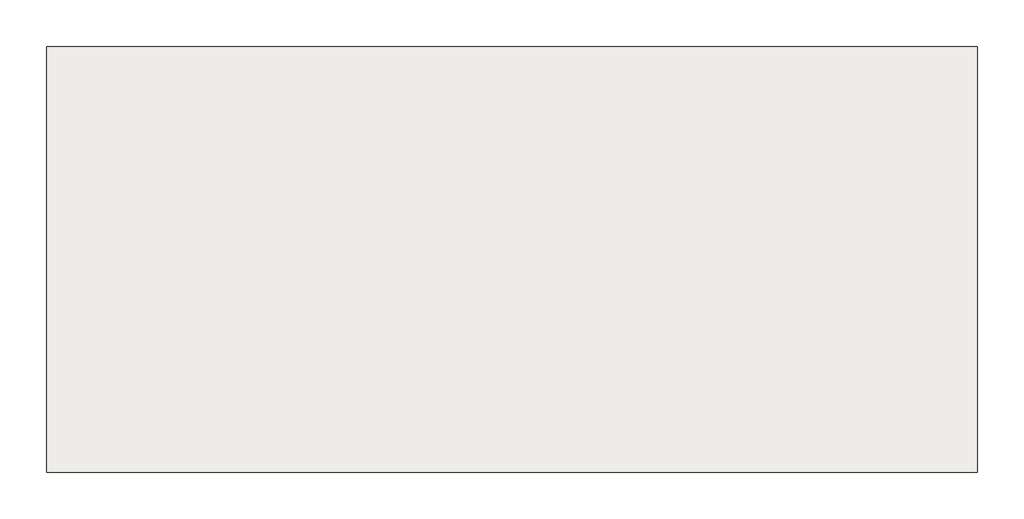
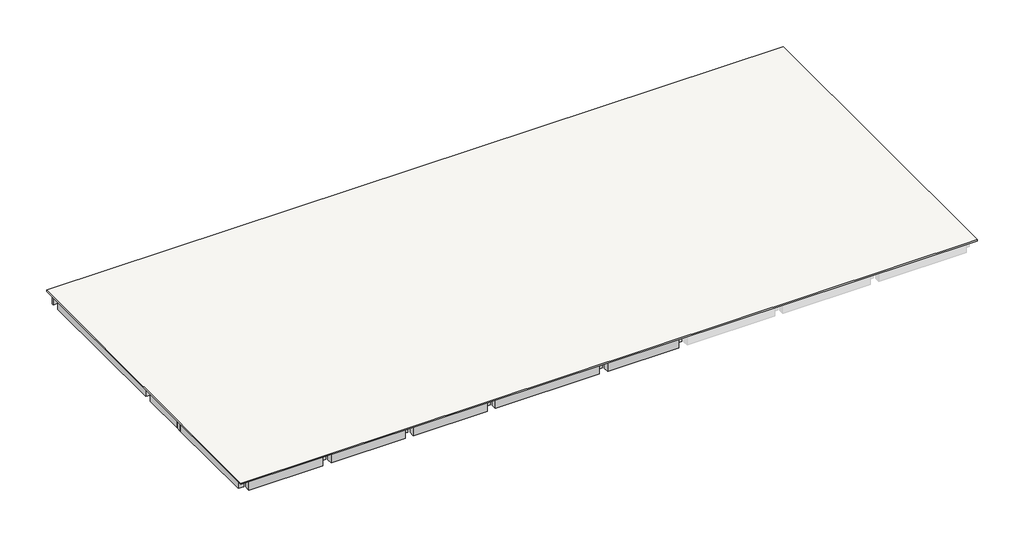
# One storey, part 1 of 2: 29 beams, 1 roof.
"""IFC4 building model written with IfcOpenShell, lengths in millimetres."""

from ifc_helpers import new_model, si_unit, frame, origin, place, context, project, spatial, polyline, outline, extrude, faceted_brep, element, save

model = new_model("IFC4")

# Units and contexts
model_context = context("Model", 3, world=origin())
ifc_project = project(units=[si_unit("LENGTHUNIT", "METRE", prefix="MILLI")], contexts=[model_context])

# Site, building, storey
site = spatial("IfcSite", under=ifc_project)
building = spatial("IfcBuilding", under=site)
storey = spatial("IfcBuildingStorey", under=building, Name="TOC", Elevation=7650.0)

# Beams
placement = place(None, origin())
element("IfcBeam", 1, ObjectType="RC Beam_Rectangular : H_SB_ACB_B400xH900", at=placement, inside=storey, context=model_context, shape_type="Brep", body=[
    faceted_brep([(224.7, 12116.5208589, 7500.0), (224.7, 12116.5208589, 6750.0), (5624.7, 12116.5208589, 6750.0), (5624.7, 12116.5208589, 7500.0), (5724.7, 12116.5208589, 7500.0), (6124.7, 12116.5208589, 7500.0), (6124.7, 12116.5208589, 7549.0), (5724.7, 12116.5208589, 7549.0), (124.7, 12116.5208589, 7549.0), (-275.3, 12116.5208589, 7549.0), (-275.3, 12116.5208589, 7500.0), (124.7, 12116.5208589, 7500.0), (224.7, 12516.5208589, 6750.0), (5624.7, 12516.5208589, 6750.0), (224.7, 12516.5208589, 7500.0), (124.7, 12516.5208589, 7500.0), (-275.3, 12516.5208589, 7500.0), (-275.3, 12516.5208589, 7549.0), (124.7, 12516.5208589, 7549.0), (5724.7, 12516.5208589, 7549.0), (6124.7, 12516.5208589, 7549.0), (6124.7, 12516.5208589, 7500.0), (5724.7, 12516.5208589, 7500.0), (5624.7, 12516.5208589, 7500.0)], [[[0, 1, 2, 3, 4, 5, 6, 7, 8, 9, 10, 11]], [[1, 12, 13, 2]], [[12, 14, 15, 16, 17, 18, 19, 20, 21, 22, 23, 13]], [[1, 0, 14, 12]], [[0, 11, 10, 16, 15, 14]], [[23, 3, 2, 13]], [[3, 23, 22, 21, 5, 4]], [[9, 8, 7, 6, 20, 19, 18, 17]], [[9, 17, 16, 10]], [[20, 6, 5, 21]]]),
])
element("IfcBeam", 2, ObjectType="RC Beam_Rectangular : H_SB_ACB_B400xH900", at=placement, inside=storey, context=model_context, shape_type="Brep", body=[
    faceted_brep([(6224.7, 12116.5208589, 7500.0), (6224.7, 12116.5208589, 6750.0), (11624.7, 12116.5208589, 6750.0), (11624.7, 12116.5208589, 7500.0), (11724.7, 12116.5208589, 7500.0), (12124.7, 12116.5208589, 7500.0), (12124.7, 12116.5208589, 7549.0), (11724.7, 12116.5208589, 7549.0), (6124.7, 12116.5208589, 7549.0), (6124.7, 12116.5208589, 7500.0), (6224.7, 12516.5208589, 6750.0), (11624.7, 12516.5208589, 6750.0), (6224.7, 12516.5208589, 7500.0), (6124.7, 12516.5208589, 7500.0), (6124.7, 12516.5208589, 7549.0), (11724.7, 12516.5208589, 7549.0), (12124.7, 12516.5208589, 7549.0), (12124.7, 12516.5208589, 7500.0), (11724.7, 12516.5208589, 7500.0), (11624.7, 12516.5208589, 7500.0)], [[[0, 1, 2, 3, 4, 5, 6, 7, 8, 9]], [[1, 10, 11, 2]], [[10, 12, 13, 14, 15, 16, 17, 18, 19, 11]], [[1, 0, 12, 10]], [[0, 9, 13, 12]], [[19, 3, 2, 11]], [[3, 19, 18, 17, 5, 4]], [[8, 7, 6, 16, 15, 14]], [[16, 6, 5, 17]], [[8, 14, 13, 9]]]),
])
element("IfcBeam", 3, ObjectType="RC Beam_Rectangular : H_SB_ACB_B400xH900", at=placement, inside=storey, context=model_context, shape_type="Brep", body=[
    faceted_brep([(12224.7, 12116.5208589, 7500.0), (12224.7, 12116.5208589, 6750.0), (17624.7, 12116.5208589, 6750.0), (17624.7, 12116.5208589, 7500.0), (17724.7, 12116.5208589, 7500.0), (18124.7, 12116.5208589, 7500.0), (18124.7, 12116.5208589, 7549.0), (17724.7, 12116.5208589, 7549.0), (12124.7, 12116.5208589, 7549.0), (12124.7, 12116.5208589, 7500.0), (12224.7, 12516.5208589, 6750.0), (17624.7, 12516.5208589, 6750.0), (12224.7, 12516.5208589, 7500.0), (12124.7, 12516.5208589, 7500.0), (12124.7, 12516.5208589, 7549.0), (17724.7, 12516.5208589, 7549.0), (18124.7, 12516.5208589, 7549.0), (18124.7, 12516.5208589, 7500.0), (17724.7, 12516.5208589, 7500.0), (17624.7, 12516.5208589, 7500.0)], [[[0, 1, 2, 3, 4, 5, 6, 7, 8, 9]], [[1, 10, 11, 2]], [[10, 12, 13, 14, 15, 16, 17, 18, 19, 11]], [[1, 0, 12, 10]], [[0, 9, 13, 12]], [[19, 3, 2, 11]], [[3, 19, 18, 17, 5, 4]], [[8, 7, 6, 16, 15, 14]], [[16, 6, 5, 17]], [[8, 14, 13, 9]]]),
])
element("IfcBeam", 4, ObjectType="RC Beam_Rectangular : H_SB_ACB_B400xH900", at=placement, inside=storey, context=model_context, shape_type="Brep", body=[
    faceted_brep([(26324.7, 12116.5208589, 7549.0), (25924.7, 12116.5208589, 7549.0), (18124.7, 12116.5208589, 7549.0), (18124.7, 12116.5208589, 7500.0), (18224.7, 12116.5208589, 7500.0), (18224.7, 12116.5208589, 6750.0), (25924.7, 12116.5208589, 6750.0), (26324.7, 12116.5208589, 6750.0), (26324.7, 12516.5208589, 6750.0), (18224.7, 12516.5208589, 6750.0), (25924.7, 12516.5208589, 6750.0), (18124.7, 12516.5208589, 7549.0), (25924.7, 12516.5208589, 7549.0), (26324.7, 12516.5208589, 7549.0), (18224.7, 12516.5208589, 7500.0), (18124.7, 12516.5208589, 7500.0)], [[[0, 1, 2, 3, 4, 5, 6, 7]], [[8, 7, 6, 5, 9, 10]], [[11, 12, 13, 8, 10, 9, 14, 15]], [[4, 14, 9, 5]], [[14, 4, 3, 15]], [[2, 1, 0, 13, 12, 11]], [[7, 8, 13, 0]], [[2, 11, 15, 3]]]),
])
element("IfcBeam", 5, ObjectType="RC Beam_Rectangular : H_SB_ACB_B400xH900", at=placement, inside=storey, context=model_context, shape_type="Brep", body=[
    faceted_brep([(32124.7, 12116.5208589, 6750.0), (32124.7, 12116.5208589, 7549.0), (31724.7, 12116.5208589, 7549.0), (26324.7, 12116.5208589, 7549.0), (26324.7, 12116.5208589, 6750.0), (31724.7, 12116.5208589, 6750.0), (32124.7, 12516.5208589, 6750.0), (26324.7, 12516.5208589, 6750.0), (31724.7, 12516.5208589, 6750.0), (32124.7, 12516.5208589, 7549.0), (26324.7, 12516.5208589, 7549.0), (31724.7, 12516.5208589, 7549.0)], [[[0, 1, 2, 3, 4, 5]], [[6, 0, 5, 4, 7, 8]], [[9, 6, 8, 7, 10, 11]], [[1, 9, 11, 10, 3, 2]], [[0, 6, 9, 1]], [[4, 3, 10, 7]]]),
])
element("IfcBeam", 6, ObjectType="RC Beam_Rectangular : H_SB_ACB_B400xH900", at=placement, inside=storey, context=model_context, shape_type="Brep", body=[
    faceted_brep([(-275.3, 8216.5208589, 6750.0), (124.7, 8216.5208589, 6750.0), (5724.7, 8216.5208589, 6750.0), (6124.7, 8216.5208589, 6750.0), (6124.7, 8216.5208589, 7549.0), (5724.7, 8216.5208589, 7549.0), (124.7, 8216.5208589, 7549.0), (-275.3, 8216.5208589, 7549.0), (-275.3, 8616.5208589, 6750.0), (124.7, 8616.5208589, 6750.0), (5724.7, 8616.5208589, 6750.0), (6124.7, 8616.5208589, 6750.0), (-275.3, 8616.5208589, 7549.0), (124.7, 8616.5208589, 7549.0), (5724.7, 8616.5208589, 7549.0), (6124.7, 8616.5208589, 7549.0)], [[[0, 1, 2, 3, 4, 5, 6, 7]], [[0, 8, 9, 10, 11, 3, 2, 1]], [[11, 10, 9, 8, 12, 13, 14, 15]], [[7, 6, 5, 4, 15, 14, 13, 12]], [[8, 0, 7, 12]], [[3, 11, 15, 4]]]),
])
element("IfcBeam", 7, ObjectType="RC Beam_Rectangular : H_SB_ACB_B400xH900", at=placement, inside=storey, context=model_context, shape_type="Brep", body=[
    faceted_brep([(12124.7, 8216.5208589, 6750.0), (12124.7, 8216.5208589, 7549.0), (11724.7, 8216.5208589, 7549.0), (6124.7, 8216.5208589, 7549.0), (6124.7, 8216.5208589, 6750.0), (11724.7, 8216.5208589, 6750.0), (12124.7, 8616.5208589, 6750.0), (6124.7, 8616.5208589, 6750.0), (11724.7, 8616.5208589, 6750.0), (12124.7, 8616.5208589, 7549.0), (6124.7, 8616.5208589, 7549.0), (11724.7, 8616.5208589, 7549.0)], [[[0, 1, 2, 3, 4, 5]], [[6, 0, 5, 4, 7, 8]], [[9, 6, 8, 7, 10, 11]], [[1, 9, 11, 10, 3, 2]], [[0, 6, 9, 1]], [[4, 3, 10, 7]]]),
])
element("IfcBeam", 8, ObjectType="RC Beam_Rectangular : H_SB_ACB_B400xH900", at=placement, inside=storey, context=model_context, shape_type="Brep", body=[
    faceted_brep([(18124.7, 8216.5208589, 6750.0), (18124.7, 8216.5208589, 7549.0), (17724.7, 8216.5208589, 7549.0), (12124.7, 8216.5208589, 7549.0), (12124.7, 8216.5208589, 6750.0), (17724.7, 8216.5208589, 6750.0), (18124.7, 8616.5208589, 6750.0), (12124.7, 8616.5208589, 6750.0), (17724.7, 8616.5208589, 6750.0), (18124.7, 8616.5208589, 7549.0), (12124.7, 8616.5208589, 7549.0), (17724.7, 8616.5208589, 7549.0)], [[[0, 1, 2, 3, 4, 5]], [[6, 0, 5, 4, 7, 8]], [[9, 6, 8, 7, 10, 11]], [[1, 9, 11, 10, 3, 2]], [[0, 6, 9, 1]], [[4, 3, 10, 7]]]),
])
element("IfcBeam", 9, ObjectType="RC Beam_Rectangular : H_SB_ACB_B400xH900", at=placement, inside=storey, context=model_context, shape_type="Brep", body=[
    faceted_brep([(26324.7, 8216.5208589, 7549.0), (25924.7, 8216.5208589, 7549.0), (18124.7, 8216.5208589, 7549.0), (18124.7, 8216.5208589, 6750.0), (25824.7, 8216.5208589, 6750.0), (25824.7, 8216.5208589, 7500.0), (25924.7, 8216.5208589, 7500.0), (26324.7, 8216.5208589, 7500.0), (18124.7, 8616.5208589, 6750.0), (25824.7, 8616.5208589, 6750.0), (18124.7, 8616.5208589, 7549.0), (25924.7, 8616.5208589, 7549.0), (26324.7, 8616.5208589, 7549.0), (26324.7, 8616.5208589, 7500.0), (25924.7, 8616.5208589, 7500.0), (25824.7, 8616.5208589, 7500.0)], [[[0, 1, 2, 3, 4, 5, 6, 7]], [[3, 8, 9, 4]], [[10, 11, 12, 13, 14, 15, 9, 8]], [[15, 5, 4, 9]], [[5, 15, 14, 13, 7, 6]], [[2, 1, 0, 12, 11, 10]], [[12, 0, 7, 13]], [[3, 2, 10, 8]]]),
])
element("IfcBeam", 10, ObjectType="RC Beam_Rectangular : H_SB_ACB_B400xH900", at=placement, inside=storey, context=model_context, shape_type="Brep", body=[
    faceted_brep([(26424.7, 8216.5208589, 7500.0), (26424.7, 8216.5208589, 6750.0), (31624.7, 8216.5208589, 6750.0), (31624.7, 8216.5208589, 7500.0), (31724.7, 8216.5208589, 7500.0), (32124.7, 8216.5208589, 7500.0), (32124.7, 8216.5208589, 7549.0), (31724.7, 8216.5208589, 7549.0), (26324.7, 8216.5208589, 7549.0), (26324.7, 8216.5208589, 7500.0), (26424.7, 8616.5208589, 6750.0), (31624.7, 8616.5208589, 6750.0), (26424.7, 8616.5208589, 7500.0), (26324.7, 8616.5208589, 7500.0), (26324.7, 8616.5208589, 7549.0), (31724.7, 8616.5208589, 7549.0), (32124.7, 8616.5208589, 7549.0), (32124.7, 8616.5208589, 7500.0), (31724.7, 8616.5208589, 7500.0), (31624.7, 8616.5208589, 7500.0)], [[[0, 1, 2, 3, 4, 5, 6, 7, 8, 9]], [[1, 10, 11, 2]], [[10, 12, 13, 14, 15, 16, 17, 18, 19, 11]], [[1, 0, 12, 10]], [[0, 9, 13, 12]], [[19, 3, 2, 11]], [[3, 19, 18, 17, 5, 4]], [[8, 7, 6, 16, 15, 14]], [[16, 6, 5, 17]], [[8, 14, 13, 9]]]),
])
element("IfcBeam", 11, ObjectType="RC Beam_Rectangular : H_SB_ACB_B400xH900", at=placement, inside=storey, context=model_context, shape_type="Brep", body=[
    faceted_brep([(224.7, 416.5208589, 7500.0), (224.7, 416.5208589, 6750.0), (5624.7, 416.5208589, 6750.0), (5624.7, 416.5208589, 7500.0), (6124.7, 416.5208589, 7500.0), (6124.7, 416.5208589, 7549.0), (-275.3, 416.5208589, 7549.0), (-275.3, 416.5208589, 7500.0), (224.7, 816.5208589, 6750.0), (5624.7, 816.5208589, 6750.0), (224.7, 816.5208589, 7500.0), (124.7, 816.5208589, 7500.0), (-275.3, 816.5208589, 7500.0), (-275.3, 816.5208589, 7549.0), (124.7, 816.5208589, 7549.0), (5724.7, 816.5208589, 7549.0), (6124.7, 816.5208589, 7549.0), (6124.7, 816.5208589, 7500.0), (5724.7, 816.5208589, 7500.0), (5624.7, 816.5208589, 7500.0)], [[[0, 1, 2, 3, 4, 5, 6, 7]], [[1, 8, 9, 2]], [[8, 10, 11, 12, 13, 14, 15, 16, 17, 18, 19, 9]], [[8, 1, 0, 10]], [[12, 11, 10, 0, 7]], [[19, 3, 2, 9]], [[3, 19, 18, 17, 4]], [[6, 5, 16, 15, 14, 13]], [[6, 13, 12, 7]], [[16, 5, 4, 17]]]),
])
element("IfcBeam", 12, ObjectType="RC Beam_Rectangular : H_SB_ACB_B400xH900", at=placement, inside=storey, context=model_context, shape_type="Brep", body=[
    faceted_brep([(6224.7, 416.5208589, 7500.0), (6224.7, 416.5208589, 6750.0), (11624.7, 416.5208589, 6750.0), (11624.7, 416.5208589, 7500.0), (12124.7, 416.5208589, 7500.0), (12124.7, 416.5208589, 7549.0), (6124.7, 416.5208589, 7549.0), (6124.7, 416.5208589, 7500.0), (6224.7, 816.5208589, 6750.0), (11624.7, 816.5208589, 6750.0), (6224.7, 816.5208589, 7500.0), (6124.7, 816.5208589, 7500.0), (6124.7, 816.5208589, 7549.0), (11724.7, 816.5208589, 7549.0), (12124.7, 816.5208589, 7549.0), (12124.7, 816.5208589, 7500.0), (11724.7, 816.5208589, 7500.0), (11624.7, 816.5208589, 7500.0)], [[[0, 1, 2, 3, 4, 5, 6, 7]], [[1, 8, 9, 2]], [[8, 10, 11, 12, 13, 14, 15, 16, 17, 9]], [[8, 1, 0, 10]], [[11, 10, 0, 7]], [[17, 3, 2, 9]], [[3, 17, 16, 15, 4]], [[6, 5, 14, 13, 12]], [[14, 5, 4, 15]], [[6, 12, 11, 7]]]),
])
element("IfcBeam", 13, ObjectType="RC Beam_Rectangular : H_SB_ACB_B400xH900", at=placement, inside=storey, context=model_context, shape_type="Brep", body=[
    faceted_brep([(12224.7, 416.5208589, 7500.0), (12224.7, 416.5208589, 6750.0), (17624.7, 416.5208589, 6750.0), (17624.7, 416.5208589, 7500.0), (18124.7, 416.5208589, 7500.0), (18124.7, 416.5208589, 7549.0), (12124.7, 416.5208589, 7549.0), (12124.7, 416.5208589, 7500.0), (12224.7, 816.5208589, 6750.0), (17624.7, 816.5208589, 6750.0), (12224.7, 816.5208589, 7500.0), (12124.7, 816.5208589, 7500.0), (12124.7, 816.5208589, 7549.0), (17724.7, 816.5208589, 7549.0), (18124.7, 816.5208589, 7549.0), (18124.7, 816.5208589, 7500.0), (17724.7, 816.5208589, 7500.0), (17624.7, 816.5208589, 7500.0)], [[[0, 1, 2, 3, 4, 5, 6, 7]], [[1, 8, 9, 2]], [[8, 10, 11, 12, 13, 14, 15, 16, 17, 9]], [[8, 1, 0, 10]], [[11, 10, 0, 7]], [[17, 3, 2, 9]], [[3, 17, 16, 15, 4]], [[6, 5, 14, 13, 12]], [[14, 5, 4, 15]], [[6, 12, 11, 7]]]),
])
element("IfcBeam", 14, ObjectType="RC Beam_Rectangular : H_SB_ACB_B400xH900", at=placement, inside=storey, context=model_context, shape_type="Brep", body=[
    faceted_brep([(18224.7, 416.5208589, 7500.0), (18224.7, 416.5208589, 6750.0), (25824.7, 416.5208589, 6750.0), (25824.7, 416.5208589, 7500.0), (26324.7, 416.5208589, 7500.0), (26324.7, 416.5208589, 7549.0), (18124.7, 416.5208589, 7549.0), (18124.7, 416.5208589, 7500.0), (18224.7, 816.5208589, 6750.0), (25824.7, 816.5208589, 6750.0), (18224.7, 816.5208589, 7500.0), (18124.7, 816.5208589, 7500.0), (18124.7, 816.5208589, 7549.0), (25924.7, 816.5208589, 7549.0), (26324.7, 816.5208589, 7549.0), (26324.7, 816.5208589, 7500.0), (25924.7, 816.5208589, 7500.0), (25824.7, 816.5208589, 7500.0)], [[[0, 1, 2, 3, 4, 5, 6, 7]], [[1, 8, 9, 2]], [[8, 10, 11, 12, 13, 14, 15, 16, 17, 9]], [[8, 1, 0, 10]], [[11, 10, 0, 7]], [[17, 3, 2, 9]], [[3, 17, 16, 15, 4]], [[6, 5, 14, 13, 12]], [[14, 5, 4, 15]], [[6, 12, 11, 7]]]),
])
element("IfcBeam", 15, ObjectType="RC Beam_Rectangular : H_SB_ACB_B400xH900", at=placement, inside=storey, context=model_context, shape_type="Brep", body=[
    faceted_brep([(26424.7, 416.5208589, 7500.0), (26424.7, 416.5208589, 6750.0), (31624.7, 416.5208589, 6750.0), (31624.7, 416.5208589, 7500.0), (32124.7, 416.5208589, 7500.0), (32124.7, 416.5208589, 7549.0), (26324.7, 416.5208589, 7549.0), (26324.7, 416.5208589, 7500.0), (26424.7, 816.5208589, 6750.0), (31624.7, 816.5208589, 6750.0), (26424.7, 816.5208589, 7500.0), (26324.7, 816.5208589, 7500.0), (26324.7, 816.5208589, 7549.0), (31724.7, 816.5208589, 7549.0), (32124.7, 816.5208589, 7549.0), (32124.7, 816.5208589, 7500.0), (31724.7, 816.5208589, 7500.0), (31624.7, 816.5208589, 7500.0)], [[[0, 1, 2, 3, 4, 5, 6, 7]], [[1, 8, 9, 2]], [[8, 10, 11, 12, 13, 14, 15, 16, 17, 9]], [[8, 1, 0, 10]], [[11, 10, 0, 7]], [[17, 3, 2, 9]], [[3, 17, 16, 15, 4]], [[6, 5, 14, 13, 12]], [[14, 5, 4, 15]], [[6, 12, 11, 7]]]),
])
element("IfcBeam", 16, ObjectType="RC Beam_Rectangular : H_SB_ACB_B400xH900", at=placement, inside=storey, context=model_context, shape_type="SweptSolid", body=[
    extrude(outline(polyline([(8216.5208589, 7549.0), (8216.5208589, 6750.0), (916.5208589, 6750.0), (916.5208589, 7500.0), (816.5208589, 7500.0), (816.5208589, 7549.0), (8216.5208589, 7549.0)])), frame((-275.3, 0.0, 0.0), z_axis=(1.0, 0.0, 0.0), x_axis=(0.0, 1.0, 0.0)), (0.0, 0.0, 1.0), 400.0),
])
element("IfcBeam", 17, ObjectType="RC Beam_Rectangular : H_SB_ACB_B400xH900", at=placement, inside=storey, context=model_context, shape_type="SweptSolid", body=[
    extrude(outline(polyline([(8616.5208589, 7549.0), (12116.5208589, 7549.0), (12116.5208589, 7500.0), (12016.5208589, 7500.0), (12016.5208589, 6750.0), (8616.5208589, 6750.0), (8616.5208589, 7549.0)])), frame((-275.3, 0.0, 0.0), z_axis=(1.0, 0.0, 0.0), x_axis=(0.0, 1.0, 0.0)), (0.0, 0.0, 1.0), 400.0),
])
element("IfcBeam", 18, ObjectType="RC Beam_Rectangular : H_SB_ACB_B400xH900", at=placement, inside=storey, context=model_context, shape_type="Brep", body=[
    faceted_brep([(124.7, 24429.2208589, 6750.0), (-275.3, 24429.2208589, 6750.0), (-275.3, 24429.2208589, 7549.0), (124.7, 24429.2208589, 7549.0), (124.7, 12616.5208589, 7500.0), (124.7, 12616.5208589, 6750.0), (124.7, 23716.5208589, 6750.0), (124.7, 23716.5208589, 7500.0), (124.7, 23816.5208589, 7500.0), (124.7, 24216.5208589, 7500.0), (124.7, 24316.5208589, 7500.0), (124.7, 24316.5208589, 6750.0), (124.7, 24216.5208589, 7549.0), (124.7, 23816.5208589, 7549.0), (124.7, 12516.5208589, 7549.0), (124.7, 12516.5208589, 7500.0), (-275.3, 24316.5208589, 6750.0), (-275.3, 12616.5208589, 6750.0), (-275.3, 12616.5208589, 7500.0), (-275.3, 12516.5208589, 7500.0), (-275.3, 12516.5208589, 7549.0), (-275.3, 24316.5208589, 7500.0), (-275.3, 23716.5208589, 7500.0), (-275.3, 23716.5208589, 6750.0)], [[[0, 1, 2, 3]], [[4, 5, 6, 7, 8, 9, 10, 11, 0, 3, 12, 13, 14, 15]], [[1, 0, 11, 16]], [[17, 18, 19, 20, 2, 1, 16, 21, 22, 23]], [[19, 15, 14, 20]], [[5, 4, 18, 17]], [[4, 15, 19, 18]], [[22, 7, 6, 23]], [[7, 22, 21, 10, 9, 8]], [[3, 2, 20, 14, 13, 12]], [[10, 21, 16, 11]], [[5, 17, 23, 6]]]),
])
element("IfcBeam", 19, ObjectType="RC Beam_Rectangular : H_SB_ACB_B400xH900", at=placement, inside=storey, context=model_context, shape_type="SweptSolid", body=[
    extrude(outline(polyline([(8216.5208589, 7549.0), (8216.5208589, 6750.0), (916.5208589, 6750.0), (916.5208589, 7500.0), (816.5208589, 7500.0), (816.5208589, 7549.0), (8216.5208589, 7549.0)])), frame((5724.7, 0.0, 0.0), z_axis=(1.0, 0.0, 0.0), x_axis=(0.0, 1.0, 0.0)), (0.0, 0.0, 1.0), 400.0),
])
element("IfcBeam", 20, ObjectType="RC Beam_Rectangular : H_SB_ACB_B400xH900", at=placement, inside=storey, context=model_context, shape_type="SweptSolid", body=[
    extrude(outline(polyline([(8616.5208589, 6750.0), (8616.5208589, 7549.0), (12116.5208589, 7549.0), (12116.5208589, 7500.0), (12016.5208589, 7500.0), (12016.5208589, 6750.0), (8616.5208589, 6750.0)])), frame((5724.7, 0.0, 0.0), z_axis=(1.0, 0.0, 0.0), x_axis=(0.0, 1.0, 0.0)), (0.0, 0.0, 1.0), 400.0),
])
element("IfcBeam", 21, ObjectType="RC Beam_Rectangular : H_SB_ACB_B400xH900", at=placement, inside=storey, context=model_context, shape_type="Brep", body=[
    faceted_brep([(6124.7, 24429.2208589, 6750.0), (5724.7, 24429.2208589, 6750.0), (5724.7, 24429.2208589, 7549.0), (6124.7, 24429.2208589, 7549.0), (6124.7, 12616.5208589, 7500.0), (6124.7, 12616.5208589, 6750.0), (6124.7, 23716.5208589, 6750.0), (6124.7, 23716.5208589, 7500.0), (6124.7, 23816.5208589, 7500.0), (6124.7, 24216.5208589, 7500.0), (6124.7, 24316.5208589, 7500.0), (6124.7, 24316.5208589, 6750.0), (6124.7, 24216.5208589, 7549.0), (6124.7, 23816.5208589, 7549.0), (6124.7, 12516.5208589, 7549.0), (6124.7, 12516.5208589, 7500.0), (5724.7, 24316.5208589, 6750.0), (5724.7, 24316.5208589, 7500.0), (5724.7, 24216.5208589, 7500.0), (5724.7, 23816.5208589, 7500.0), (5724.7, 23716.5208589, 7500.0), (5724.7, 23716.5208589, 6750.0), (5724.7, 12616.5208589, 6750.0), (5724.7, 12616.5208589, 7500.0), (5724.7, 12516.5208589, 7500.0), (5724.7, 12516.5208589, 7549.0), (5724.7, 23816.5208589, 7549.0), (5724.7, 24216.5208589, 7549.0)], [[[0, 1, 2, 3]], [[4, 5, 6, 7, 8, 9, 10, 11, 0, 3, 12, 13, 14, 15]], [[1, 0, 11, 16]], [[2, 1, 16, 17, 18, 19, 20, 21, 22, 23, 24, 25, 26, 27]], [[24, 15, 14, 25]], [[5, 4, 23, 22]], [[4, 15, 24, 23]], [[20, 7, 6, 21]], [[7, 20, 19, 18, 17, 10, 9, 8]], [[3, 2, 27, 26, 25, 14, 13, 12]], [[10, 17, 16, 11]], [[5, 22, 21, 6]]]),
])
element("IfcBeam", 22, ObjectType="RC Beam_Rectangular : H_SB_ACB_B400xH900", at=placement, inside=storey, context=model_context, shape_type="SweptSolid", body=[
    extrude(outline(polyline([(8216.5208589, 7549.0), (8216.5208589, 6750.0), (916.5208589, 6750.0), (916.5208589, 7500.0), (816.5208589, 7500.0), (816.5208589, 7549.0), (8216.5208589, 7549.0)])), frame((11724.7, 0.0, 0.0), z_axis=(1.0, 0.0, 0.0), x_axis=(0.0, 1.0, 0.0)), (0.0, 0.0, 1.0), 400.0),
])
element("IfcBeam", 23, ObjectType="RC Beam_Rectangular : H_SB_ACB_B400xH900", at=placement, inside=storey, context=model_context, shape_type="SweptSolid", body=[
    extrude(outline(polyline([(8616.5208589, 6750.0), (8616.5208589, 7549.0), (12116.5208589, 7549.0), (12116.5208589, 7500.0), (12016.5208589, 7500.0), (12016.5208589, 6750.0), (8616.5208589, 6750.0)])), frame((11724.7, 0.0, 0.0), z_axis=(1.0, 0.0, 0.0), x_axis=(0.0, 1.0, 0.0)), (0.0, 0.0, 1.0), 400.0),
])
element("IfcBeam", 24, ObjectType="RC Beam_Rectangular : H_SB_ACB_B400xH900", at=placement, inside=storey, context=model_context, shape_type="SweptSolid", body=[
    extrude(outline(polyline([(8216.5208589, 7549.0), (8216.5208589, 6750.0), (916.5208589, 6750.0), (916.5208589, 7500.0), (816.5208589, 7500.0), (816.5208589, 7549.0), (8216.5208589, 7549.0)])), frame((17724.7, 0.0, 0.0), z_axis=(1.0, 0.0, 0.0), x_axis=(0.0, 1.0, 0.0)), (0.0, 0.0, 1.0), 400.0),
])
element("IfcBeam", 25, ObjectType="RC Beam_Rectangular : H_SB_ACB_B400xH900", at=placement, inside=storey, context=model_context, shape_type="SweptSolid", body=[
    extrude(outline(polyline([(8616.5208589, 6750.0), (8616.5208589, 7549.0), (12116.5208589, 7549.0), (12116.5208589, 7500.0), (12016.5208589, 7500.0), (12016.5208589, 6750.0), (8616.5208589, 6750.0)])), frame((17724.7, 0.0, 0.0), z_axis=(1.0, 0.0, 0.0), x_axis=(0.0, 1.0, 0.0)), (0.0, 0.0, 1.0), 400.0),
])
element("IfcBeam", 26, ObjectType="RC Beam_Rectangular : H_SB_ACB_B400xH900", at=placement, inside=storey, context=model_context, shape_type="SweptSolid", body=[
    extrude(outline(polyline([(8116.5208589, 7500.0), (8116.5208589, 6750.0), (916.5208589, 6750.0), (916.5208589, 7500.0), (816.5208589, 7500.0), (816.5208589, 7549.0), (8216.5208589, 7549.0), (8216.5208589, 7500.0), (8116.5208589, 7500.0)])), frame((25924.7, 0.0, 0.0), z_axis=(1.0, 0.0, 0.0), x_axis=(0.0, 1.0, 0.0)), (0.0, 0.0, 1.0), 400.0),
])
element("IfcBeam", 27, ObjectType="RC Beam_Rectangular : H_SB_ACB_B400xH900", at=placement, inside=storey, context=model_context, shape_type="SweptSolid", body=[
    extrude(outline(polyline([(12116.5208589, 7549.0), (12116.5208589, 6750.0), (8716.5208589, 6750.0), (8716.5208589, 7500.0), (8616.5208589, 7500.0), (8616.5208589, 7549.0), (12116.5208589, 7549.0)])), frame((25924.7, 0.0, 0.0), z_axis=(1.0, 0.0, 0.0), x_axis=(0.0, 1.0, 0.0)), (0.0, 0.0, 1.0), 400.0),
])
element("IfcBeam", 28, ObjectType="RC Beam_Rectangular : H_SB_ACB_B400xH900", at=placement, inside=storey, context=model_context, shape_type="SweptSolid", body=[
    extrude(outline(polyline([(8116.5208589, 7500.0), (8116.5208589, 6750.0), (916.5208589, 6750.0), (916.5208589, 7500.0), (816.5208589, 7500.0), (816.5208589, 7549.0), (8216.5208589, 7549.0), (8216.5208589, 7500.0), (8116.5208589, 7500.0)])), frame((31724.7, 0.0, 0.0), z_axis=(1.0, 0.0, 0.0), x_axis=(0.0, 1.0, 0.0)), (0.0, 0.0, 1.0), 400.0),
])
element("IfcBeam", 29, ObjectType="RC Beam_Rectangular : H_SB_ACB_B400xH900", at=placement, inside=storey, context=model_context, shape_type="SweptSolid", body=[
    extrude(outline(polyline([(12116.5208589, 7549.0), (12116.5208589, 6750.0), (8716.5208589, 6750.0), (8716.5208589, 7500.0), (8616.5208589, 7500.0), (8616.5208589, 7549.0), (12116.5208589, 7549.0)])), frame((31724.7, 0.0, 0.0), z_axis=(1.0, 0.0, 0.0), x_axis=(0.0, 1.0, 0.0)), (0.0, 0.0, 1.0), 400.0),
])

# Roof
element("IfcRoof", 30, ObjectType="H_RF_AMF_RC Roof Finish_WP_Insulation_Protection", at=placement, inside=storey, context=model_context, shape_type="SweptSolid", body=[
    extrude(outline(polyline([(53324.7, 24816.5208589), (53324.7, 216.5208589), (-475.3, 216.5208589), (-475.3, 24816.5208589), (53324.7, 24816.5208589)])), frame((0.0, 0.0, 7549.0), z_axis=(0.0, 0.0, 1.0), x_axis=(1.0, 0.0, 0.0)), (0.0, 0.0, 1.0), 101.0),
])

save(model, "model.ifc")

# Revit data of these elements
# Type "RC Beam_Rectangular : H_SB_ACB_B400xH900"
#   중앙부 하부근 = ""
#   중앙부 상부근 = ""
#   중앙부 보조근 = ""
#   중앙부 늑근 = ""
#   외단부 하부근 = ""
#   외단부 상부근 = ""
#   외단부 보조근 = ""
#   외단부 늑근 = ""
#   부호 = "TG3"
#   내단부 하부근 = ""
#   내단부 상부근 = ""
#   내단부 보조근 = ""
#   내단부 늑근 = ""
#   ALL 하부근 = "3-D20"
#   ALL 상부근 = "3-D20"
#   ALL 보조근 = ""
#   ALL 늑근 = "2-D10 @120"
#   Width = 400.000 mm
#   Height = 900.000 mm
#   Length [instance default] = 1524.000 mm
#   b = 400.000 mm
#   h = 900.000 mm
#   hec_material3 [instance default] = none
#   hec_material2 [instance default] = none
#   hec_material1 [instance default] = none
#   Structural Material [instance default] = none
#   Assembly Code = ""
# Type "H_RF_AMF_RC Roof Finish_WP_Insulation_Protection"
#   Layers, outside or top first: 50.000 mm no material (function 4); 0.000 mm no material (function 100); 50.000 mm no material (function 3); 1.000 mm no material (function 2)
# Elements 1, 2, 3, 4, 5, 6, 7, 8, 9, 10, 11, 12, 13, 14, 15, 16, 17, 18, 19, 20, 21, 22, 23, 24, 25, 26, 27, 28, 29 (IfcBeam, "RC Beam_Rectangular : H_SB_ACB_B400xH900")
#   hec_material3 = none
#   hec_material2 = none
#   hec_material1 = none
#   Structural Material = none
#   Phase Created = New Construction
# Element 30 (IfcRoof, "H_RF_AMF_RC Roof Finish_WP_Insulation_Protection")
#   Mark = "RF1"
#   Roof Style Name = "Lightweight Concrete(Slope)+Insulation+Waterproofing+Gravel"
#   Roof Ref. = ""
#   Roof Base Material = "Concrete Slab"
#   Roof Finish_1 = "Light-Weight Concrete Screed (Slope 1%)"
#   Roof Finish_2 = ""
#   Roof Finish_3 = "Rigid Extruded Polystyrene Foam Insulation(XPS)"
#   Roof Finish_4 = "Waterproofing Membrane-EPDM(or Equivalent)"
#   Roof Finish_5 = "Gravel for Roof"
#   built-in parameter 1001705 = 25.0984 (stored number, unit not read)
#   built-in parameter 1001701 = -0.331365 (stored number, unit not read)
#   built-in parameter 1001710 = 33615
#   Roof Style = RF13
#   Phase Created = New Construction
#   Materials on its faces: "Default Roof"
# Materials
#   "Default Roof": class "Miscellaneous", colour RGB 80 80 80, transparency 0
